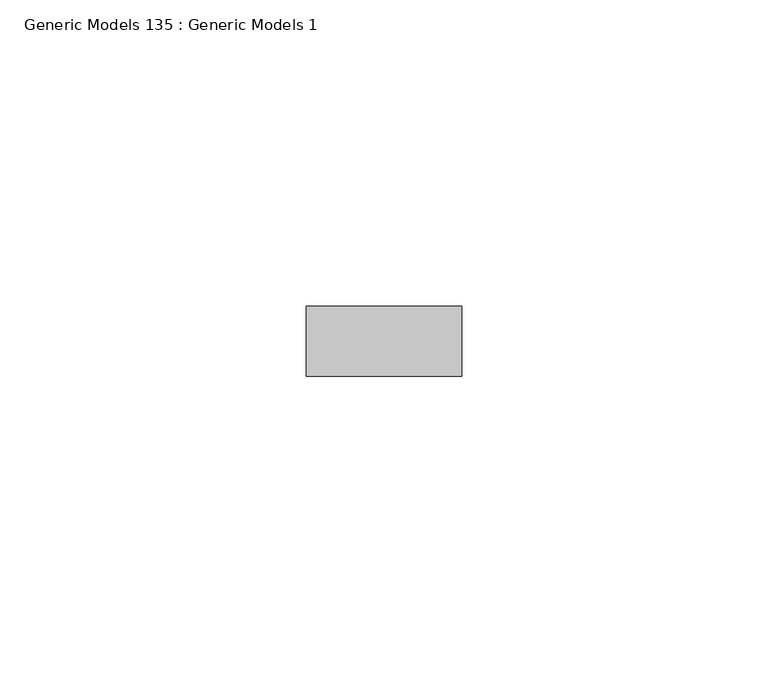
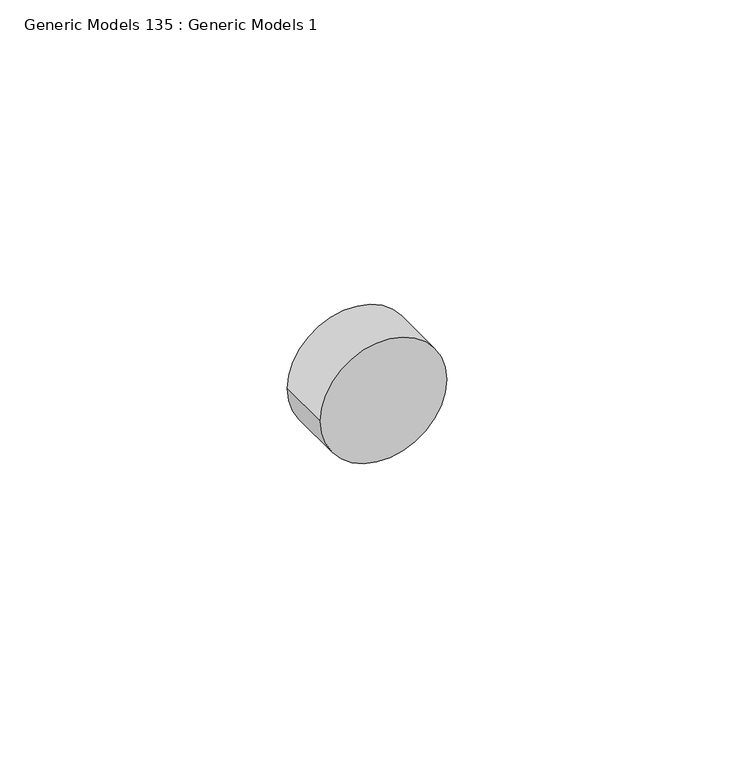
"""IFC4 building model written with IfcOpenShell, lengths in millimetres: proxy geometry, Generic Models 135 : Generic Models 1."""

from ifc_helpers import new_model, si_unit, point, frame, frame_2d, origin, place, context, project, spatial, circle_curve, trimmed, segment, composite_curve, outline, extrude, source, transform, mapped, element, save


def generic_models_135_generic_models_1_c43b58a6(model_context):
    return source(origin(), model_context, "Body", "SweptSolid", [
        extrude(outline(composite_curve([segment(trimmed(circle_curve(frame_2d((38717.9805939, 8135.7346014)), 12.7), [point((38717.9805939, 8148.4346014))], [point((38717.9805939, 8123.0346014))], False, "CARTESIAN"), True, "CONTINUOUS"), segment(trimmed(circle_curve(frame_2d((38717.9805939, 8135.7346014)), 12.7), [point((38717.9805939, 8123.0346014))], [point((38717.9805939, 8148.4346014))], False, "CARTESIAN"), True, "CONTINUOUS")], self_intersect=False)), frame((0.0, 1836.9202358, 0.0), z_axis=(0.0, 1.0, 0.0), x_axis=(0.0, 0.0, 1.0)), (0.0, 0.0, 1.0), 11.4464372),
    ])


if __name__ == "__main__":
    model = new_model("IFC4")
    model_context = context("Model", 3, world=origin())
    ifc_project = project(units=[si_unit("LENGTHUNIT", "METRE", prefix="MILLI")], contexts=[model_context])
    site = spatial("IfcSite", under=ifc_project)
    building = spatial("IfcBuilding", under=site)
    placement = place(None, origin())
    generic_models_135_generic_models_1_shape = generic_models_135_generic_models_1_c43b58a6(model_context)
    element("IfcBuildingElementProxy", 1, Name="Generic Models 135 : Generic Models 1", ObjectType="Generic Models 135 : Generic Models 1", at=placement, inside=building, context=model_context, shape_type="MappedRepresentation", body=[
        mapped(generic_models_135_generic_models_1_shape, transform((0.0, 0.0, 0.0), x_axis=(1.0, 0.0, 0.0), y_axis=(0.0, 1.0, 0.0), z_axis=(0.0, 0.0, 1.0))),
    ])
    save(model, "model.ifc")

# Revit data of these elements
# Element 1 (IfcBuildingElementProxy, "Generic Models 135 : Generic Models 1")
#   Materials on its faces: "S.S. LAG BOLT - SEE STRUCT. DWGS"
# Materials
#   "S.S. LAG BOLT - SEE STRUCT. DWGS": class "Generic", colour RGB 120 120 120, transparency 0, Cost = 0
